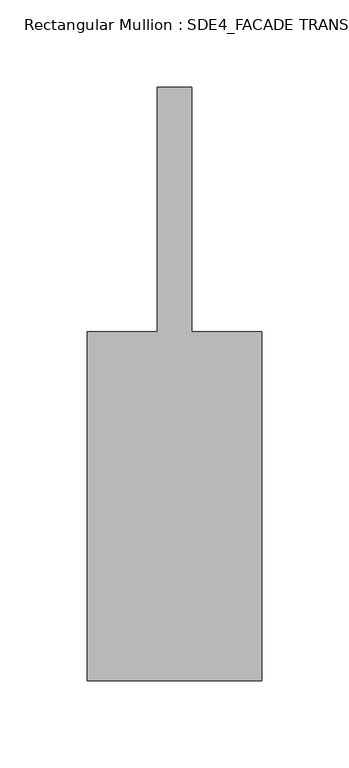
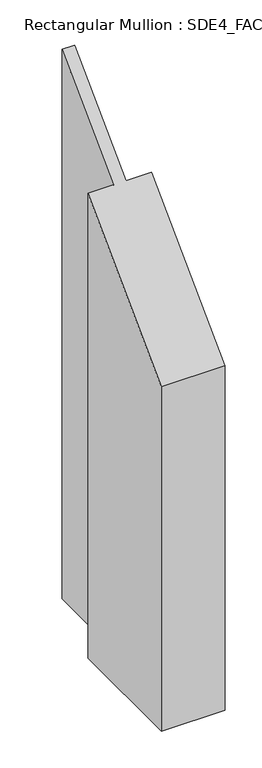
"""IFC4 building model written with IfcOpenShell, lengths in millimetres: member geometry, Rectangular Mullion : SDE4_FACADE TRANSOM TYPE 1."""

from ifc_helpers import new_model, si_unit, origin, place, context, project, spatial, faceted_brep, source, transform, mapped, element, save


def rectangular_mullion_sde4_facade_transom_type_1_7dbe6f18(model_context):
    return source(origin(), model_context, "Body", "Brep", [
        faceted_brep([(50.0, -132.5, -704.7378664), (-50.0, -132.5, -704.7378664), (-50.0, 67.5, -704.7378664), (-10.0, 67.5, -704.7378664), (-10.0, 207.5, -704.7378664), (10.0, 207.5, -704.7378664), (10.0, 67.5, -704.7378664), (50.0, 67.5, -704.7378664), (50.0, 67.5, 67.5), (50.0, -132.5, -132.5), (10.0, 67.5, 67.5), (10.0, 207.5, 207.5), (-10.0, 207.5, 207.5), (-10.0, 67.5, 67.5), (-50.0, 67.5, 67.5), (-50.0, -132.5, -132.5)], [[[0, 1, 2, 3, 4, 5, 6, 7]], [[8, 9, 0, 7]], [[10, 8, 7, 6]], [[11, 10, 6, 5]], [[12, 11, 5, 4]], [[13, 12, 4, 3]], [[14, 13, 3, 2]], [[15, 14, 2, 1]], [[9, 15, 1, 0]], [[9, 8, 10, 11, 12, 13, 14, 15]]]),
    ])


if __name__ == "__main__":
    model = new_model("IFC4")
    model_context = context("Model", 3, world=origin())
    ifc_project = project(units=[si_unit("LENGTHUNIT", "METRE", prefix="MILLI")], contexts=[model_context])
    site = spatial("IfcSite", under=ifc_project)
    building = spatial("IfcBuilding", under=site)
    placement = place(None, origin())
    rectangular_mullion_sde4_facade_transom_type_1_shape = rectangular_mullion_sde4_facade_transom_type_1_7dbe6f18(model_context)
    element("IfcMember", 1, ObjectType="Rectangular Mullion : SDE4_FACADE TRANSOM TYPE 1", at=placement, inside=building, context=model_context, shape_type="MappedRepresentation", body=[
        mapped(rectangular_mullion_sde4_facade_transom_type_1_shape, transform((0.0, 0.0, 0.0), x_axis=(1.0, 0.0, 0.0), y_axis=(0.0, 1.0, 0.0), z_axis=(0.0, 0.0, 1.0))),
    ])
    save(model, "model.ifc")

# Revit data of these elements
# Type "Rectangular Mullion : SDE4_FACADE TRANSOM TYPE 1"
#   built-in parameter 1007322 = 1.11549 (stored number, unit not read)
#   built-in parameter 1007321 = 0.164042 (stored number, unit not read)
#   built-in parameter 1007320 = 0.164042 (stored number, unit not read)
